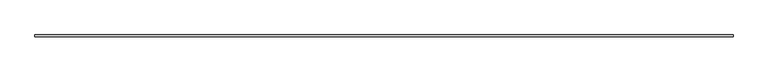
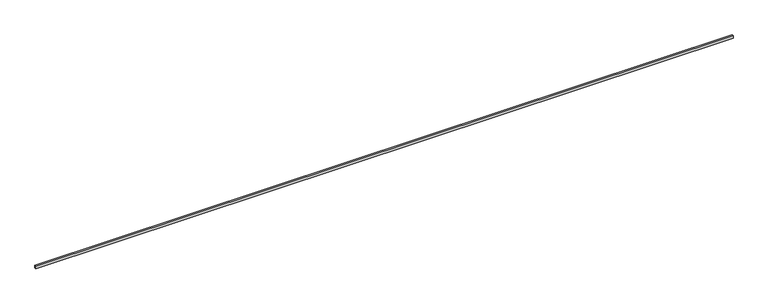
"""IFC4 building model written with IfcOpenShell, lengths in millimetres: proxy geometry, Generic Models 3:Generic Models 2:312240:Generic Models 2:312240 : Generic Models 3:Generic Models 2:312240:13 : Generic Models 3:Generic Models 2:312240:Generic Models 2:312240 : Generic Models 3:Generic Models 2:312240:300533."""

from ifc_helpers import new_model, si_unit, frame, origin, place, context, project, spatial, polyline, outline, extrude, source, transform, mapped, element, save


def generic_models_6f53a7f9(model_context):
    return source(origin(), model_context, "Body", "SweptSolid", [
        extrude(outline(polyline([(-579008.485222, 1189.8500487), (-579010.3823183, 1190.3583741), (-579011.9127678, 1190.0885146), (-579013.3913841, 1188.6098983), (-579013.3913841, 1197.8637896), (-579007.0413841, 1197.8637896), (-579007.0413841, 1188.8390625), (-579008.485222, 1189.8500487)])), frame((590317.0242239, 0.0, 0.0), z_axis=(1.0, 0.0, 0.0), x_axis=(0.0, 1.0, 0.0)), (0.0, 0.0, 1.0), 2438.4),
    ])


if __name__ == "__main__":
    model = new_model("IFC4")
    model_context = context("Model", 3, world=origin())
    ifc_project = project(units=[si_unit("LENGTHUNIT", "METRE", prefix="MILLI")], contexts=[model_context])
    site = spatial("IfcSite", under=ifc_project)
    building = spatial("IfcBuilding", under=site)
    placement = place(None, origin())
    generic_models_shape = generic_models_6f53a7f9(model_context)
    element("IfcBuildingElementProxy", 1, Name="Generic Models 3:Generic Models 2:312240:Generic Models 2:312240 : Generic Models 3:Generic Models 2:312240:13 : Generic Models 3:Generic Models 2:312240:Generic Models 2:312240 : Generic Models 3:Generic Models 2:312240:300533", ObjectType="Generic Models 3:Generic Models 2:312240:Generic Models 2:312240 : Generic Models 3:Generic Models 2:312240:13 : Generic Models 3:Generic Models 2:312240:Generic Models 2:312240 : Generic Models 3:Generic Models 2:312240:300533", at=placement, inside=building, context=model_context, shape_type="MappedRepresentation", body=[
        mapped(generic_models_shape, transform((0.0, 0.0, 0.0), x_axis=(1.0, 0.0, 0.0), y_axis=(0.0, 1.0, 0.0), z_axis=(0.0, 0.0, 1.0))),
    ])
    save(model, "model.ifc")

# Revit data of these elements
# Type "Generic Models 3:Generic Models 2:312240:Generic Models 2:312240 : Generic Models 3:Generic Models 2:312240:13 : Generic Models 3:Generic Models 2:312240:Generic Models 2:312240 : Generic Models 3:Generic Models 2:312240:300533"
#   NameOverride = "Generic Models 3:Generic Models 2:312240:Generic Models 2:312240 : Generic Models 3:Generic Models 2:312240:300533"
#   ObjectTypeOverride = "Generic Models 2:312240 : Generic Models 3:Generic Models 2:312240"
#   Reference = "Generic Models 2"
#   Tag = "300533"
# Element 1 (IfcBuildingElementProxy, "Generic Models 3:Generic Models 2:312240:Generic Models 2:312240 : Generic Models 3:Generic Models 2:312240:13 : Generic Models 3:Generic Models 2:312240:Generic Models 2:312240 : Generic Models 3:Generic Models 2:312240:300533")
#   Materials on its faces: "SILICONE SEALANT"
# Materials
#   "SILICONE SEALANT": class "Generic", colour RGB 221 221 221, transparency 0, Cost = 0
